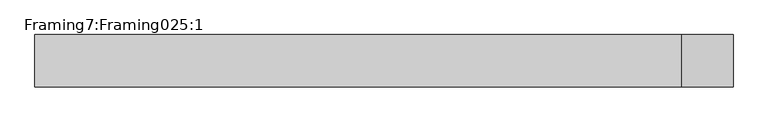
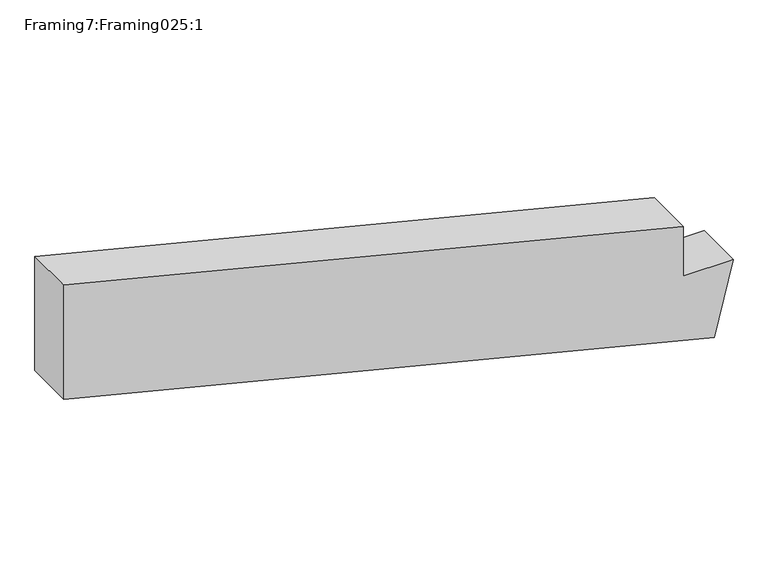
"""IFC4 building model written with IfcOpenShell, lengths in millimetres: proxy geometry, Framing7:Framing025:1 : Framing7:Framing025:286338."""

from ifc_helpers import new_model, si_unit, frame, origin, place, context, project, spatial, polyline, outline, extrude, source, transform, mapped, element, save


def framing7_framing025_1_c5c29cc2(model_context):
    return source(origin(), model_context, "Body", "SweptSolid", [
        extrude(outline(polyline([(111678.1362587, 15130.8894286), (111908.8006385, 15187.4083443), (111908.8006385, 15036.8413595), (112067.5842581, 15036.8413595), (112537.4873042, 13157.0903708), (112170.6516785, 13157.0903708), (111678.1362587, 15130.8894286)])), frame((0.0, -14445.349577, 0.0), z_axis=(0.0, 1.0, 0.0), x_axis=(0.0, 0.0, 1.0)), (0.0, 0.0, 1.0), 152.4),
    ])


if __name__ == "__main__":
    model = new_model("IFC4")
    model_context = context("Model", 3, world=origin())
    ifc_project = project(units=[si_unit("LENGTHUNIT", "METRE", prefix="MILLI")], contexts=[model_context])
    site = spatial("IfcSite", under=ifc_project)
    building = spatial("IfcBuilding", under=site)
    placement = place(None, origin())
    framing7_framing025_1_shape = framing7_framing025_1_c5c29cc2(model_context)
    element("IfcBuildingElementProxy", 1, Name="Framing7:Framing025:1 : Framing7:Framing025:286338", ObjectType="Framing7:Framing025:1 : Framing7:Framing025:286338", at=placement, inside=building, context=model_context, shape_type="MappedRepresentation", body=[
        mapped(framing7_framing025_1_shape, transform((0.0, 0.0, 0.0), x_axis=(1.0, 0.0, 0.0), y_axis=(0.0, 1.0, 0.0), z_axis=(0.0, 0.0, 1.0))),
    ])
    save(model, "model.ifc")

# Revit data of these elements
# Type "Framing7:Framing025:1 : Framing7:Framing025:286338"
#   NameOverride = "Framing7:Framing025:286338"
#   ObjectTypeOverride = "Framing7:Framing025"
#   Reference = "Framing025"
#   Category = "Generic Models"
#   Tag = "286338"
# Element 1 (IfcBuildingElementProxy, "Framing7:Framing025:1 : Framing7:Framing025:286338")
#   Materials on its faces: "WOOD FRAMING (SEE STRUCT DWGS)"
# Materials
#   "WOOD FRAMING (SEE STRUCT DWGS)": class "Unassigned", colour RGB 224 188 168, transparency 0, Cost = 0
